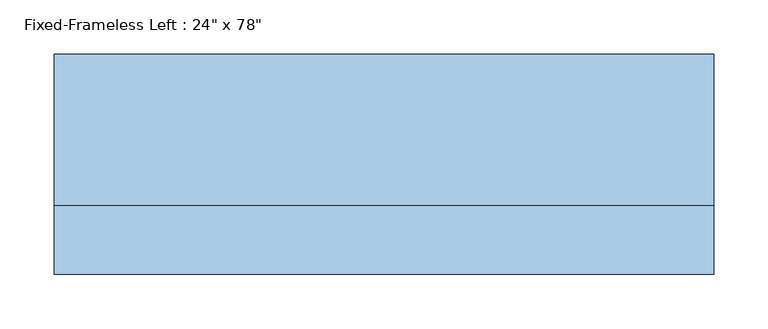
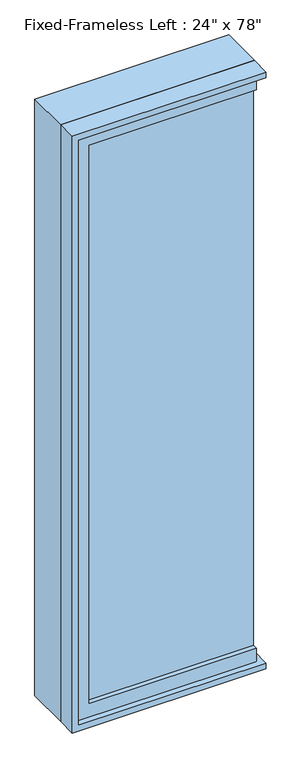
"""IFC4 building model written with IfcOpenShell, lengths in millimetres: window geometry."""

import ifcopenshell
import ifcopenshell.guid

model = None  # the IFC model being written
_history = None  # IfcOwnerHistory: only IFC2X3 demands one
_inside = {}  # id of a spatial element -> (the spatial element, [elements in it])
_under = {}  # id of a project, library or spatial element -> (it, [spatial elements below it])
_declared = {}  # id of a project -> (the project, [libraries it declares])
_typed = {}  # id of a type object -> (the type object, [elements of that type])
_made_of = {}  # id of a material, layer set ... -> (it, [elements and type objects made of it])


def new_model(schema):
    """Start an empty IFC model of exactly this schema.

    Asked for "IFC4X3", IfcOpenShell would pick the latest addendum, in which some entities
    have other attributes; the version numbers below select the first issue.
    IFC2X3 requires an IfcOwnerHistory on every rooted entity: one is made here for all.
    """
    global model, _history
    if schema == "IFC4X3":
        model = ifcopenshell.file(schema_version=(4, 3, 0, 0))
    else:
        model = ifcopenshell.file(schema=schema)
    _inside.clear()
    _under.clear()
    _declared.clear()
    _typed.clear()
    _made_of.clear()
    _history = None
    if model.schema == "IFC2X3":
        org = make("IfcOrganization", Name="unknown")
        user = make(
            "IfcPersonAndOrganization",
            ThePerson=make("IfcPerson", FamilyName="unknown"),
            TheOrganization=org,
        )
        app = make(
            "IfcApplication",
            ApplicationDeveloper=org,
            Version="unknown",
            ApplicationFullName="unknown",
            ApplicationIdentifier="unknown",
        )
        _history = make(
            "IfcOwnerHistory",
            OwningUser=user,
            OwningApplication=app,
            ChangeAction="ADDED",
            CreationDate=0,
        )
    return model


def make(cls, **values):
    """One entity of the class cls with the attributes given. An attribute that is None is left unset."""
    return model.create_entity(
        cls, **{name: value for name, value in values.items() if value is not None}
    )


def rooted(cls, **values):
    """An entity with a GlobalId (a new one), such as an element, a storey or a relation."""
    return make(cls, GlobalId=ifcopenshell.guid.new(), OwnerHistory=_history, **values)


def si_unit(unit_type, name, prefix=None):
    """IfcSIUnit, for example si_unit("LENGTHUNIT", "METRE", prefix="MILLI")."""
    return make("IfcSIUnit", UnitType=unit_type, Prefix=prefix, Name=name)


def assignment(units):
    """IfcUnitAssignment: the units of a project."""
    return None if units is None else make("IfcUnitAssignment", Units=units)


def point(xyz):
    """IfcCartesianPoint."""
    return None if xyz is None else make("IfcCartesianPoint", Coordinates=xyz)


def direction(xyz):
    """IfcDirection."""
    return None if xyz is None else make("IfcDirection", DirectionRatios=xyz)


def frame(location, z_axis=None, x_axis=None):
    """IfcAxis2Placement3D, a coordinate frame: its origin and axes. An axis left out is left unset."""
    return make(
        "IfcAxis2Placement3D",
        Location=point(location),
        Axis=direction(z_axis),
        RefDirection=direction(x_axis),
    )


def origin():
    """The frame at (0, 0, 0) with its axes left unset."""
    return frame((0.0, 0.0, 0.0))


def place(relative_to, where):
    """IfcLocalPlacement: puts the frame where relative to a parent placement (None: the world)."""
    return make(
        "IfcLocalPlacement", PlacementRelTo=relative_to, RelativePlacement=where
    )


def context(
    kind, dimensions, precision=None, world=None, true_north=None, identifier=None
):
    """IfcGeometricRepresentationContext, for example the 3D "Model" context."""
    return make(
        "IfcGeometricRepresentationContext",
        ContextIdentifier=identifier,
        ContextType=kind,
        CoordinateSpaceDimension=dimensions,
        Precision=precision,
        WorldCoordinateSystem=world,
        TrueNorth=true_north,
    )


def project(units=None, contexts=None):
    """IfcProject with its units and contexts."""
    return rooted(
        "IfcProject",
        Name="project",
        RepresentationContexts=contexts,
        UnitsInContext=assignment(units),
    )


def spatial(cls, under=None, at=None, **own):
    """A site, building, storey or space (cls), placed at a placement, below another one or the project."""
    s = rooted(cls, ObjectPlacement=at, **own)
    if under is not None:
        _under.setdefault(under.id(), (under, []))[1].append(s)
    return s


def polyline(points):
    """IfcPolyline through the points."""
    return make("IfcPolyline", Points=[point(p) for p in points])


def outline(outer, holes=None, kind="AREA"):
    """IfcArbitraryClosedProfileDef: a profile drawn as a closed curve; with holes, ...WithVoids."""
    if holes is None:
        return make("IfcArbitraryClosedProfileDef", ProfileType=kind, OuterCurve=outer)
    return make(
        "IfcArbitraryProfileDefWithVoids",
        ProfileType=kind,
        OuterCurve=outer,
        InnerCurves=holes,
    )


def extrude(swept, where, along, depth):
    """IfcExtrudedAreaSolid: the profile swept, set in the frame where, extruded along a direction by depth."""
    return make(
        "IfcExtrudedAreaSolid",
        SweptArea=swept,
        Position=where,
        ExtrudedDirection=direction(along),
        Depth=depth,
    )


def shape(context_of_items, identifier, shape_type, items):
    """IfcShapeRepresentation: the items that make up one representation, for example the "Body"."""
    return make(
        "IfcShapeRepresentation",
        ContextOfItems=context_of_items,
        RepresentationIdentifier=identifier,
        RepresentationType=shape_type,
        Items=items,
    )


def source(mapping_origin, context_of_items, identifier, shape_type, items):
    """IfcRepresentationMap: a shape defined once, which mapped items show again and again."""
    return make(
        "IfcRepresentationMap",
        MappingOrigin=mapping_origin,
        MappedRepresentation=shape(context_of_items, identifier, shape_type, items),
    )


def transform(
    local_origin,
    x_axis=None,
    y_axis=None,
    z_axis=None,
    scale=None,
    scale2=None,
    scale3=None,
    uniform=True,
):
    """IfcCartesianTransformationOperator3D, or its non-uniform kind. x_axis, y_axis, z_axis: its Axis1, 2, 3."""
    if uniform:
        return make(
            "IfcCartesianTransformationOperator3D",
            Axis1=direction(x_axis),
            Axis2=direction(y_axis),
            LocalOrigin=point(local_origin),
            Scale=scale,
            Axis3=direction(z_axis),
        )
    return make(
        "IfcCartesianTransformationOperator3DnonUniform",
        Axis1=direction(x_axis),
        Axis2=direction(y_axis),
        LocalOrigin=point(local_origin),
        Scale=scale,
        Axis3=direction(z_axis),
        Scale2=scale2,
        Scale3=scale3,
    )


def mapped(mapping_source, mapping_target):
    """IfcMappedItem: shows the shape of a source again, moved by a transform."""
    return make(
        "IfcMappedItem", MappingSource=mapping_source, MappingTarget=mapping_target
    )


def made_of(thing, what):
    """Note that an element or type object is made of a material, layer set ...; save() writes the relation."""
    if what is not None:
        _made_of.setdefault(what.id(), (what, []))[1].append(thing)
    return thing


def element(
    cls,
    number,
    at=None,
    inside=None,
    cuts=None,
    type_object=None,
    material=None,
    context=None,
    identifier="Body",
    shape_type=None,
    held_by="IfcProductDefinitionShape",
    body=None,
    shapes=None,
    **own,
):
    """One element of the class cls, such as IfcWall. Its Tag is "e" and its number.

    at: its placement. inside: the storey or other place that contains it. cuts: it is an
    opening in that element (IfcRelVoidsElement). A single representation is given by context,
    identifier, shape_type and body (its items); several are given by shapes. held_by: the class
    of the entity that holds the representations. save() writes the other relations.
    """
    e = rooted(cls, Tag="e%d" % number, ObjectPlacement=at, **own)
    if body is not None:
        shapes = [shape(context, identifier, shape_type, body)]
    if shapes is not None:
        e.Representation = make(held_by, Representations=shapes)
    if inside is not None:
        _inside.setdefault(inside.id(), (inside, []))[1].append(e)
    if cuts is not None:
        rooted(
            "IfcRelVoidsElement", RelatingBuildingElement=cuts, RelatedOpeningElement=e
        )
    if type_object is not None:
        _typed.setdefault(type_object.id(), (type_object, []))[1].append(e)
    return made_of(e, material)


def aggregate(whole, parts):
    """IfcRelAggregates: a whole, such as a stair, and the parts it consists of."""
    return rooted("IfcRelAggregates", RelatingObject=whole, RelatedObjects=parts)


def save(model, path):
    """Write the relations noted so far, then the file.

    IfcRelAggregates (storeys below a building ...), IfcRelContainedInSpatialStructure (elements
    in a storey), IfcRelDefinesByType, IfcRelAssociatesMaterial and IfcRelDeclares: one each for
    every whole, place, type object, material and project.
    """
    for whole, parts in _under.values():
        aggregate(whole, parts)
    for where, things in _inside.values():
        rooted(
            "IfcRelContainedInSpatialStructure",
            RelatedElements=things,
            RelatingStructure=where,
        )
    for kind, things in _typed.values():
        rooted("IfcRelDefinesByType", RelatedObjects=things, RelatingType=kind)
    for what, things in _made_of.values():
        rooted("IfcRelAssociatesMaterial", RelatedObjects=things, RelatingMaterial=what)
    for by, libraries in _declared.values():
        rooted("IfcRelDeclares", RelatingContext=by, RelatedDefinitions=libraries)
    model.write(path)


def window_6516bf2d(model_context):
    return source(origin(), model_context, "Body", "SweptSolid", [
        extrude(outline(polyline([(247.65, -53.975), (247.65, -66.675), (-279.4, -66.675), (-279.4, -53.975), (247.65, -53.975)])), frame((0.0, 0.0, 673.1), z_axis=(0.0, 0.0, 1.0), x_axis=(1.0, 0.0, 0.0)), (0.0, 0.0, 1.0), 1854.2),
        extrude(outline(polyline([(2571.75, -323.85), (628.65, -323.85), (628.65, 247.65), (673.1, 247.65), (673.1, -279.4), (2527.3, -279.4), (2527.3, 247.65), (2571.75, 247.65), (2571.75, -323.85)])), frame((0.0, -82.55, 0.0), z_axis=(0.0, 1.0, 0.0), x_axis=(0.0, 0.0, 1.0)), (0.0, 0.0, 1.0), 44.45),
        extrude(outline(polyline([(2590.8, -342.9), (609.6, -342.9), (609.6, 266.7), (641.35, 266.7), (641.35, -311.15), (2559.05, -311.15), (2559.05, 266.7), (2590.8, 266.7), (2590.8, -342.9)])), frame((0.0, -38.1, 0.0), z_axis=(0.0, 1.0, 0.0), x_axis=(0.0, 0.0, 1.0)), (0.0, 0.0, 1.0), 139.7),
        extrude(outline(polyline([(2590.8, 266.7), (2590.8, -342.9), (609.6, -342.9), (609.6, 266.7), (628.65, 266.7), (628.65, -323.85), (2571.75, -323.85), (2571.75, 266.7), (2590.8, 266.7)])), frame((0.0, -101.6, 0.0), z_axis=(0.0, 1.0, 0.0), x_axis=(0.0, 0.0, 1.0)), (0.0, 0.0, 1.0), 63.5),
    ])


if __name__ == "__main__":
    model = new_model("IFC4")
    model_context = context("Model", 3, world=origin())
    ifc_project = project(units=[si_unit("LENGTHUNIT", "METRE", prefix="MILLI")], contexts=[model_context])
    site = spatial("IfcSite", under=ifc_project)
    building = spatial("IfcBuilding", under=site)
    placement = place(None, origin())
    window_shape = window_6516bf2d(model_context)
    element("IfcWindow", 1, ObjectType="Fixed-Frameless Left : 24\" x 78\"", at=placement, inside=building, context=model_context, shape_type="MappedRepresentation", body=[
        mapped(window_shape, transform((0.0, 0.0, 0.0), x_axis=(1.0, 0.0, 0.0), y_axis=(0.0, 1.0, 0.0), z_axis=(0.0, 0.0, 1.0))),
    ])
    save(model, "model.ifc")

# Revit data of these elements
# Type "Fixed-Frameless Left : 24\" x 78\""
#   Type Mark = "71"
#   Assembly Code = "B2020100"
#   Height = 6' - 6"
#   Default Sill Height = 2' - 0"
#   Width = 2' - 0"
#   Window Inset = 0' - 0 3/4"
#   Glass Pane Material = Glass
#   Sash Material = Sash
#   Wall Closure = (empty or 0)
# Element 1 (IfcWindow, "Fixed-Frameless Left : 24\" x 78\"")
#   Materials on its faces: "Sash", "Glass"
# Materials
#   "Glass": class "Glass", colour RGB 0 128 192, transparency 0.75
#   "Sash": class "Wood", colour RGB 224 178 126, transparency 0
